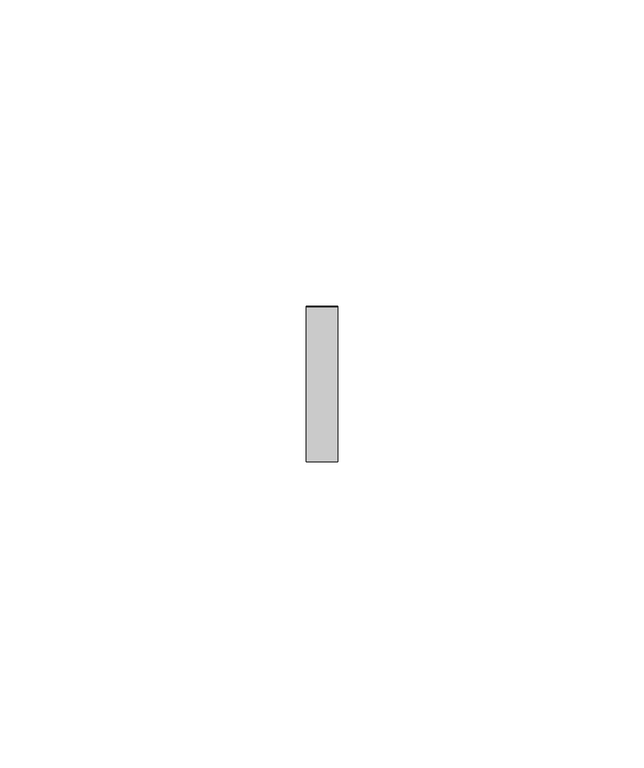
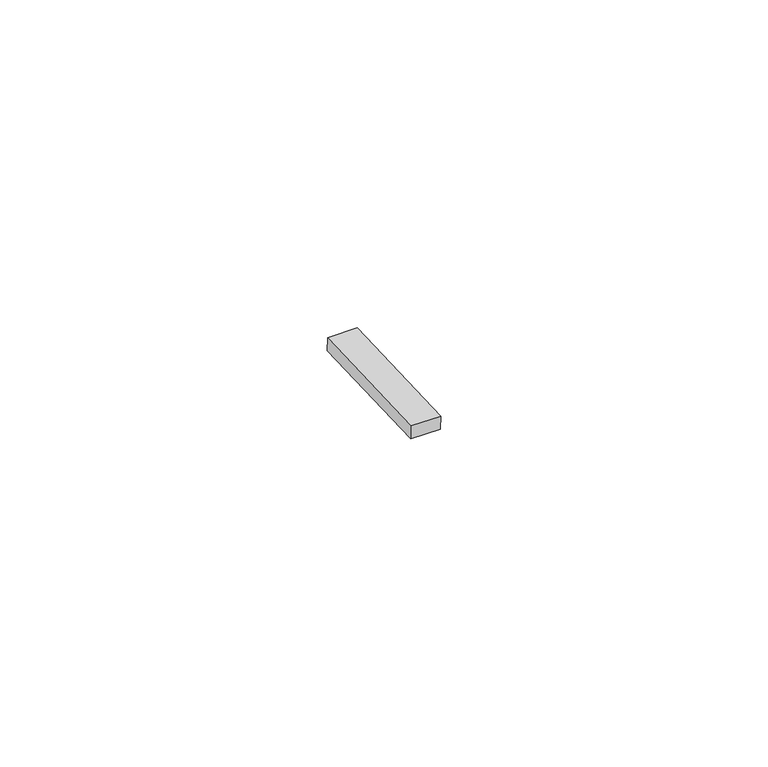
"""IFC4 building model written with IfcOpenShell, lengths in millimetres: proxy geometry, Inner panel:Inner panel:1:Inner panel:1 : Inner panel:Inner panel:300324:2:Inner panel:1:Inner panel:1 : Inner panel:Inner panel:300324:2 : Inner panel:Inner panel:1:Inner panel:1 : Inner panel:Inner panel:300324:300043:61 : Inner panel:Inner panel:1:Inner panel:1 : Inner panel:Inner panel:300324:2:Inner panel:1:Inner panel:1 : Inner panel:Inner panel:300324:2 : Inner panel:Inner panel:1:Inner panel:1 : Inner panel:Inner panel:300324:300043:308120."""

import ifcopenshell
import ifcopenshell.guid

model = None  # the IFC model being written
_history = None  # IfcOwnerHistory: only IFC2X3 demands one
_inside = {}  # id of a spatial element -> (the spatial element, [elements in it])
_under = {}  # id of a project, library or spatial element -> (it, [spatial elements below it])
_declared = {}  # id of a project -> (the project, [libraries it declares])
_typed = {}  # id of a type object -> (the type object, [elements of that type])
_made_of = {}  # id of a material, layer set ... -> (it, [elements and type objects made of it])


def new_model(schema):
    """Start an empty IFC model of exactly this schema.

    Asked for "IFC4X3", IfcOpenShell would pick the latest addendum, in which some entities
    have other attributes; the version numbers below select the first issue.
    IFC2X3 requires an IfcOwnerHistory on every rooted entity: one is made here for all.
    """
    global model, _history
    if schema == "IFC4X3":
        model = ifcopenshell.file(schema_version=(4, 3, 0, 0))
    else:
        model = ifcopenshell.file(schema=schema)
    _inside.clear()
    _under.clear()
    _declared.clear()
    _typed.clear()
    _made_of.clear()
    _history = None
    if model.schema == "IFC2X3":
        org = make("IfcOrganization", Name="unknown")
        user = make(
            "IfcPersonAndOrganization",
            ThePerson=make("IfcPerson", FamilyName="unknown"),
            TheOrganization=org,
        )
        app = make(
            "IfcApplication",
            ApplicationDeveloper=org,
            Version="unknown",
            ApplicationFullName="unknown",
            ApplicationIdentifier="unknown",
        )
        _history = make(
            "IfcOwnerHistory",
            OwningUser=user,
            OwningApplication=app,
            ChangeAction="ADDED",
            CreationDate=0,
        )
    return model


def make(cls, **values):
    """One entity of the class cls with the attributes given. An attribute that is None is left unset."""
    return model.create_entity(
        cls, **{name: value for name, value in values.items() if value is not None}
    )


def rooted(cls, **values):
    """An entity with a GlobalId (a new one), such as an element, a storey or a relation."""
    return make(cls, GlobalId=ifcopenshell.guid.new(), OwnerHistory=_history, **values)


def si_unit(unit_type, name, prefix=None):
    """IfcSIUnit, for example si_unit("LENGTHUNIT", "METRE", prefix="MILLI")."""
    return make("IfcSIUnit", UnitType=unit_type, Prefix=prefix, Name=name)


def assignment(units):
    """IfcUnitAssignment: the units of a project."""
    return None if units is None else make("IfcUnitAssignment", Units=units)


def point(xyz):
    """IfcCartesianPoint."""
    return None if xyz is None else make("IfcCartesianPoint", Coordinates=xyz)


def direction(xyz):
    """IfcDirection."""
    return None if xyz is None else make("IfcDirection", DirectionRatios=xyz)


def frame(location, z_axis=None, x_axis=None):
    """IfcAxis2Placement3D, a coordinate frame: its origin and axes. An axis left out is left unset."""
    return make(
        "IfcAxis2Placement3D",
        Location=point(location),
        Axis=direction(z_axis),
        RefDirection=direction(x_axis),
    )


def origin():
    """The frame at (0, 0, 0) with its axes left unset."""
    return frame((0.0, 0.0, 0.0))


def place(relative_to, where):
    """IfcLocalPlacement: puts the frame where relative to a parent placement (None: the world)."""
    return make(
        "IfcLocalPlacement", PlacementRelTo=relative_to, RelativePlacement=where
    )


def context(
    kind, dimensions, precision=None, world=None, true_north=None, identifier=None
):
    """IfcGeometricRepresentationContext, for example the 3D "Model" context."""
    return make(
        "IfcGeometricRepresentationContext",
        ContextIdentifier=identifier,
        ContextType=kind,
        CoordinateSpaceDimension=dimensions,
        Precision=precision,
        WorldCoordinateSystem=world,
        TrueNorth=true_north,
    )


def project(units=None, contexts=None):
    """IfcProject with its units and contexts."""
    return rooted(
        "IfcProject",
        Name="project",
        RepresentationContexts=contexts,
        UnitsInContext=assignment(units),
    )


def spatial(cls, under=None, at=None, **own):
    """A site, building, storey or space (cls), placed at a placement, below another one or the project."""
    s = rooted(cls, ObjectPlacement=at, **own)
    if under is not None:
        _under.setdefault(under.id(), (under, []))[1].append(s)
    return s


def polyline(points):
    """IfcPolyline through the points."""
    return make("IfcPolyline", Points=[point(p) for p in points])


def outline(outer, holes=None, kind="AREA"):
    """IfcArbitraryClosedProfileDef: a profile drawn as a closed curve; with holes, ...WithVoids."""
    if holes is None:
        return make("IfcArbitraryClosedProfileDef", ProfileType=kind, OuterCurve=outer)
    return make(
        "IfcArbitraryProfileDefWithVoids",
        ProfileType=kind,
        OuterCurve=outer,
        InnerCurves=holes,
    )


def extrude(swept, where, along, depth):
    """IfcExtrudedAreaSolid: the profile swept, set in the frame where, extruded along a direction by depth."""
    return make(
        "IfcExtrudedAreaSolid",
        SweptArea=swept,
        Position=where,
        ExtrudedDirection=direction(along),
        Depth=depth,
    )


def shape(context_of_items, identifier, shape_type, items):
    """IfcShapeRepresentation: the items that make up one representation, for example the "Body"."""
    return make(
        "IfcShapeRepresentation",
        ContextOfItems=context_of_items,
        RepresentationIdentifier=identifier,
        RepresentationType=shape_type,
        Items=items,
    )


def source(mapping_origin, context_of_items, identifier, shape_type, items):
    """IfcRepresentationMap: a shape defined once, which mapped items show again and again."""
    return make(
        "IfcRepresentationMap",
        MappingOrigin=mapping_origin,
        MappedRepresentation=shape(context_of_items, identifier, shape_type, items),
    )


def transform(
    local_origin,
    x_axis=None,
    y_axis=None,
    z_axis=None,
    scale=None,
    scale2=None,
    scale3=None,
    uniform=True,
):
    """IfcCartesianTransformationOperator3D, or its non-uniform kind. x_axis, y_axis, z_axis: its Axis1, 2, 3."""
    if uniform:
        return make(
            "IfcCartesianTransformationOperator3D",
            Axis1=direction(x_axis),
            Axis2=direction(y_axis),
            LocalOrigin=point(local_origin),
            Scale=scale,
            Axis3=direction(z_axis),
        )
    return make(
        "IfcCartesianTransformationOperator3DnonUniform",
        Axis1=direction(x_axis),
        Axis2=direction(y_axis),
        LocalOrigin=point(local_origin),
        Scale=scale,
        Axis3=direction(z_axis),
        Scale2=scale2,
        Scale3=scale3,
    )


def mapped(mapping_source, mapping_target):
    """IfcMappedItem: shows the shape of a source again, moved by a transform."""
    return make(
        "IfcMappedItem", MappingSource=mapping_source, MappingTarget=mapping_target
    )


def made_of(thing, what):
    """Note that an element or type object is made of a material, layer set ...; save() writes the relation."""
    if what is not None:
        _made_of.setdefault(what.id(), (what, []))[1].append(thing)
    return thing


def element(
    cls,
    number,
    at=None,
    inside=None,
    cuts=None,
    type_object=None,
    material=None,
    context=None,
    identifier="Body",
    shape_type=None,
    held_by="IfcProductDefinitionShape",
    body=None,
    shapes=None,
    **own,
):
    """One element of the class cls, such as IfcWall. Its Tag is "e" and its number.

    at: its placement. inside: the storey or other place that contains it. cuts: it is an
    opening in that element (IfcRelVoidsElement). A single representation is given by context,
    identifier, shape_type and body (its items); several are given by shapes. held_by: the class
    of the entity that holds the representations. save() writes the other relations.
    """
    e = rooted(cls, Tag="e%d" % number, ObjectPlacement=at, **own)
    if body is not None:
        shapes = [shape(context, identifier, shape_type, body)]
    if shapes is not None:
        e.Representation = make(held_by, Representations=shapes)
    if inside is not None:
        _inside.setdefault(inside.id(), (inside, []))[1].append(e)
    if cuts is not None:
        rooted(
            "IfcRelVoidsElement", RelatingBuildingElement=cuts, RelatedOpeningElement=e
        )
    if type_object is not None:
        _typed.setdefault(type_object.id(), (type_object, []))[1].append(e)
    return made_of(e, material)


def aggregate(whole, parts):
    """IfcRelAggregates: a whole, such as a stair, and the parts it consists of."""
    return rooted("IfcRelAggregates", RelatingObject=whole, RelatedObjects=parts)


def save(model, path):
    """Write the relations noted so far, then the file.

    IfcRelAggregates (storeys below a building ...), IfcRelContainedInSpatialStructure (elements
    in a storey), IfcRelDefinesByType, IfcRelAssociatesMaterial and IfcRelDeclares: one each for
    every whole, place, type object, material and project.
    """
    for whole, parts in _under.values():
        aggregate(whole, parts)
    for where, things in _inside.values():
        rooted(
            "IfcRelContainedInSpatialStructure",
            RelatedElements=things,
            RelatingStructure=where,
        )
    for kind, things in _typed.values():
        rooted("IfcRelDefinesByType", RelatedObjects=things, RelatingType=kind)
    for what, things in _made_of.values():
        rooted("IfcRelAssociatesMaterial", RelatedObjects=things, RelatingMaterial=what)
    for by, libraries in _declared.values():
        rooted("IfcRelDeclares", RelatingContext=by, RelatedDefinitions=libraries)
    model.write(path)


def generic_models_17028dce(model_context):
    return source(origin(), model_context, "Body", "SweptSolid", [
        extrude(outline(polyline([(0.0, -25.3999999), (0.0, 0.0), (5.2138089, 0.0), (5.2138089, -25.3999999), (0.0, -25.3999999)])), frame((593936.595117, -566905.6162814, 8857.0720004), z_axis=(0.0, -0.041630544712223896, 0.9991330730923502), x_axis=(-1.0, 0.0, 0.0)), (0.0, 0.0, 1.0), 2.4763745),
    ])


if __name__ == "__main__":
    model = new_model("IFC4")
    model_context = context("Model", 3, world=origin())
    ifc_project = project(units=[si_unit("LENGTHUNIT", "METRE", prefix="MILLI")], contexts=[model_context])
    site = spatial("IfcSite", under=ifc_project)
    building = spatial("IfcBuilding", under=site)
    placement = place(None, origin())
    generic_models_shape = generic_models_17028dce(model_context)
    element("IfcBuildingElementProxy", 1, Name="Inner panel:Inner panel:1:Inner panel:1 : Inner panel:Inner panel:300324:2:Inner panel:1:Inner panel:1 : Inner panel:Inner panel:300324:2 : Inner panel:Inner panel:1:Inner panel:1 : Inner panel:Inner panel:300324:300043:61 : Inner panel:Inner panel:1:Inner panel:1 : Inner panel:Inner panel:300324:2:Inner panel:1:Inner panel:1 : Inner panel:Inner panel:300324:2 : Inner panel:Inner panel:1:Inner panel:1 : Inner panel:Inner panel:300324:300043:308120", ObjectType="Inner panel:Inner panel:1:Inner panel:1 : Inner panel:Inner panel:300324:2:Inner panel:1:Inner panel:1 : Inner panel:Inner panel:300324:2 : Inner panel:Inner panel:1:Inner panel:1 : Inner panel:Inner panel:300324:300043:61 : Inner panel:Inner panel:1:Inner panel:1 : Inner panel:Inner panel:300324:2:Inner panel:1:Inner panel:1 : Inner panel:Inner panel:300324:2 : Inner panel:Inner panel:1:Inner panel:1 : Inner panel:Inner panel:300324:300043:308120", at=placement, inside=building, context=model_context, shape_type="MappedRepresentation", body=[
        mapped(generic_models_shape, transform((0.0, 0.0, 0.0), x_axis=(1.0, 0.0, 0.0), y_axis=(0.0, 1.0, 0.0), z_axis=(0.0, 0.0, 1.0))),
    ])
    save(model, "model.ifc")

# Revit data of these elements
# Type "Inner panel:Inner panel:1:Inner panel:1 : Inner panel:Inner panel:300324:2:Inner panel:1:Inner panel:1 : Inner panel:Inner panel:300324:2 : Inner panel:Inner panel:1:Inner panel:1 : Inner panel:Inner panel:300324:300043:61 : Inner panel:Inner panel:1:Inner panel:1 : Inner panel:Inner panel:300324:2:Inner panel:1:Inner panel:1 : Inner panel:Inner panel:300324:2 : Inner panel:Inner panel:1:Inner panel:1 : Inner panel:Inner panel:300324:300043:308120"
#   NameOverride = "Inner panel:Inner panel:1:Inner panel:1 : Inner panel:Inner panel:300324:2:Inner panel:1:Inner panel:1 : Inner panel:Inner panel:300324:2 : Inner panel:Inner panel:1:Inner panel:1 : Inner panel:Inner panel:300324:300043:308120"
#   ObjectTypeOverride = "Inner panel:1:Inner panel:1 : Inner panel:Inner panel:300324:2 : Inner panel:Inner panel:1:Inner panel:1 : Inner panel:Inner panel:300324:300043"
#   Reference = "Inner panel"
#   Tag = "308120"
# Element 1 (IfcBuildingElementProxy, "Inner panel:Inner panel:1:Inner panel:1 : Inner panel:Inner panel:300324:2:Inner panel:1:Inner panel:1 : Inner panel:Inner panel:300324:2 : Inner panel:Inner panel:1:Inner panel:1 : Inner panel:Inner panel:300324:300043:61 : Inner panel:Inner panel:1:Inner panel:1 : Inner panel:Inner panel:300324:2:Inner panel:1:Inner panel:1 : Inner panel:Inner panel:300324:2 : Inner panel:Inner panel:1:Inner panel:1 : Inner panel:Inner panel:300324:300043:308120")
#   Materials on its faces: "AT CLIP - 1\" WIDE NON ABSORBENT, WEATHER-RESISTANT NEOPRENE/EPDM/SBR FOAM"
# Materials
#   "AT CLIP - 1\" WIDE NON ABSORBENT, WEATHER-RESISTANT NEOPRENE/EPDM/SBR FOAM": class "Generic", colour RGB 85 85 85, transparency 0, Cost = 0
